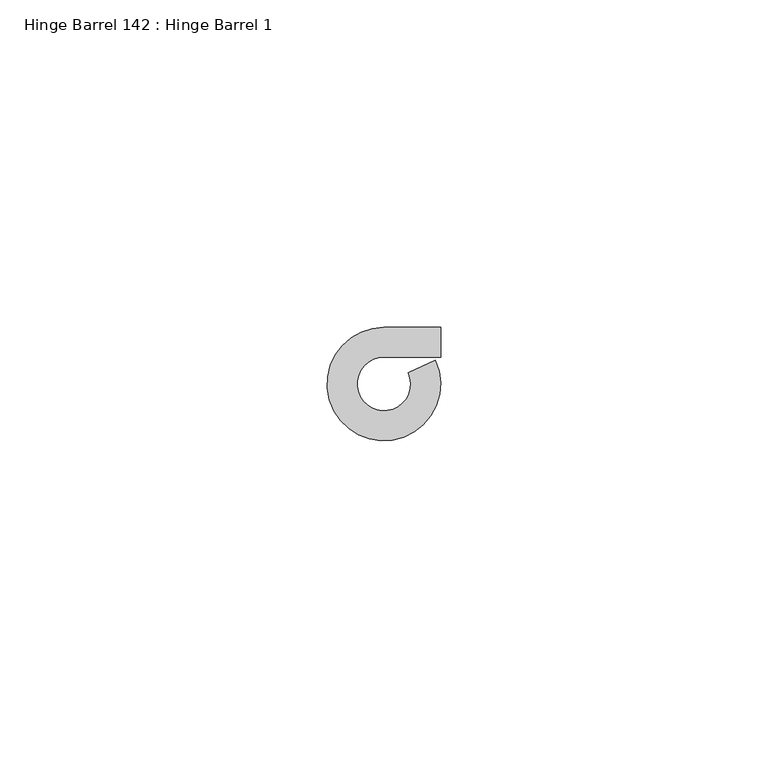
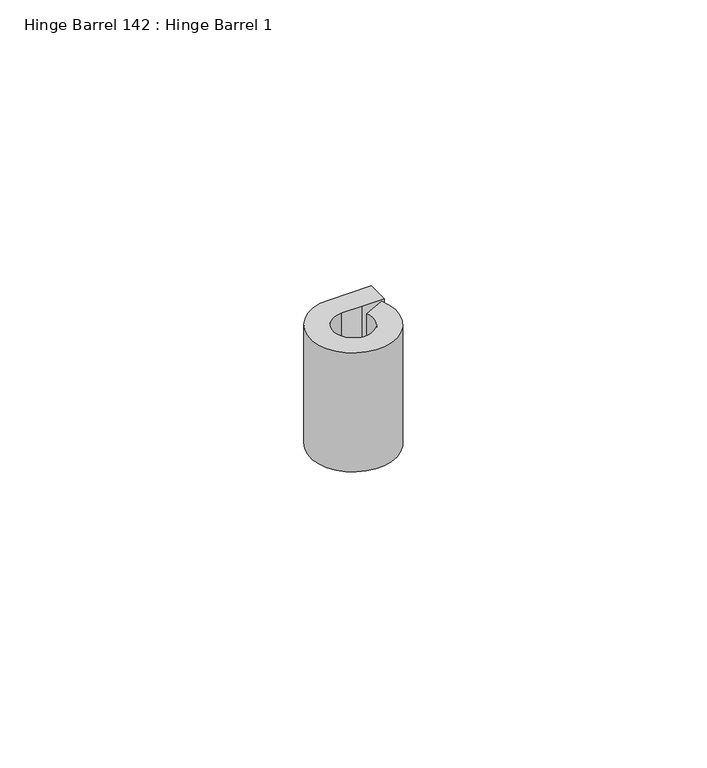
"""IFC4 building model written with IfcOpenShell, lengths in millimetres: proxy geometry, Hinge Barrel 142 : Hinge Barrel 1."""

from ifc_helpers import new_model, si_unit, point, frame, frame_2d, origin, place, context, project, spatial, polyline, circle_curve, trimmed, segment, composite_curve, outline, extrude, source, transform, mapped, element, save


def hinge_barrel_142_hinge_barrel_1_c7bfcbc0(model_context):
    return source(origin(), model_context, "Body", "SweptSolid", [
        extrude(outline(composite_curve([segment(polyline([(587323.2214739, -536306.2758841), (587319.1320739, -536306.2758841)]), True, "CONTINUOUS"), segment(trimmed(circle_curve(frame_2d((587319.1320739, -536310.3652841)), 4.0894), [point((587319.1320739, -536306.2758841))], [point((587322.8436736, -536308.6485371))], True, "CARTESIAN"), True, "CONTINUOUS"), segment(polyline([(587322.8436736, -536308.6485371), (587326.986084, -536306.7325249)]), True, "CONTINUOUS"), segment(trimmed(circle_curve(frame_2d((587319.1320739, -536310.3652841)), 8.6534625), [point((587326.986084, -536306.7325249))], [point((587319.1320739, -536301.7118216))], False, "CARTESIAN"), True, "CONTINUOUS"), segment(polyline([(587319.1320739, -536301.7118216), (587327.7934739, -536301.7118216), (587327.7934739, -536306.2758841), (587323.2214739, -536306.2758841)]), True, "CONTINUOUS")], self_intersect=False)), frame((0.0, 0.0, 1225.55), z_axis=(0.0, 0.0, 1.0), x_axis=(1.0, 0.0, 0.0)), (0.0, 0.0, 1.0), 25.4),
    ])


if __name__ == "__main__":
    model = new_model("IFC4")
    model_context = context("Model", 3, world=origin())
    ifc_project = project(units=[si_unit("LENGTHUNIT", "METRE", prefix="MILLI")], contexts=[model_context])
    site = spatial("IfcSite", under=ifc_project)
    building = spatial("IfcBuilding", under=site)
    placement = place(None, origin())
    hinge_barrel_142_hinge_barrel_1_shape = hinge_barrel_142_hinge_barrel_1_c7bfcbc0(model_context)
    element("IfcBuildingElementProxy", 1, Name="Hinge Barrel 142 : Hinge Barrel 1", ObjectType="Hinge Barrel 142 : Hinge Barrel 1", at=placement, inside=building, context=model_context, shape_type="MappedRepresentation", body=[
        mapped(hinge_barrel_142_hinge_barrel_1_shape, transform((0.0, 0.0, 0.0), x_axis=(1.0, 0.0, 0.0), y_axis=(0.0, 1.0, 0.0), z_axis=(0.0, 0.0, 1.0))),
    ])
    save(model, "model.ifc")

# Revit data of these elements
# Element 1 (IfcBuildingElementProxy, "Hinge Barrel 142 : Hinge Barrel 1")
#   Materials on its faces: "6\"X6\" WELD-ON STL BUTT HINGE"
# Materials
#   "6\"X6\" WELD-ON STL BUTT HINGE": class "Metal", colour RGB 189 187 185, transparency 0, Description = "Carbon steel", Cost = 0
